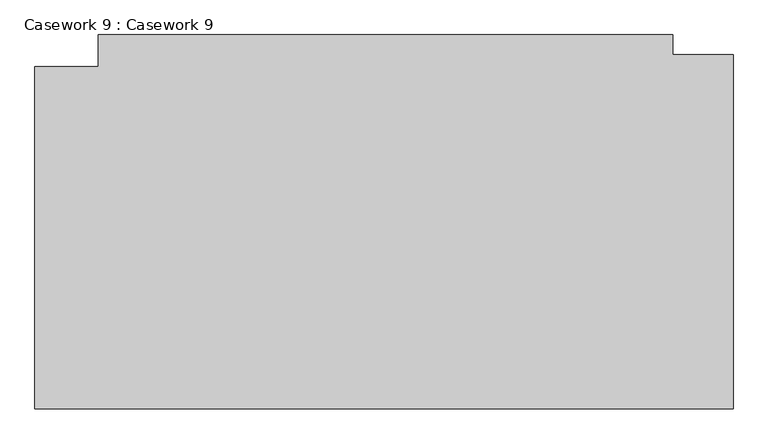
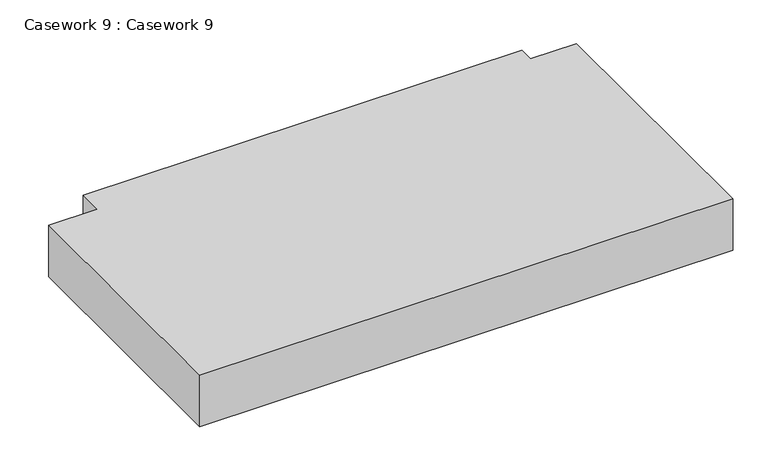
"""IFC4 building model written with IfcOpenShell, lengths in millimetres: furniture geometry, Casework 9 : Casework 9."""

from ifc_helpers import new_model, si_unit, frame, origin, place, context, project, spatial, polyline, outline, extrude, source, transform, mapped, element, save


def casework_9_casework_9_4f7e3acd(model_context):
    return source(origin(), model_context, "Body", "SweptSolid", [
        extrude(outline(polyline([(-7163.5247381, -439.3850684), (-7163.5247381, -339.3850684), (-5353.5247381, -339.3850684), (-5353.5247381, -401.8265396), (-5163.5247381, -401.8265396), (-5163.5247381, -1518.8048922), (-7363.5247381, -1518.8048922), (-7363.5247381, -439.3850684), (-7163.5247381, -439.3850684)])), frame((0.0, 0.0, -225.0091615), z_axis=(0.0, 0.0, 1.0), x_axis=(1.0, 0.0, 0.0)), (0.0, 0.0, 1.0), 225.0091615),
    ])


if __name__ == "__main__":
    model = new_model("IFC4")
    model_context = context("Model", 3, world=origin())
    ifc_project = project(units=[si_unit("LENGTHUNIT", "METRE", prefix="MILLI")], contexts=[model_context])
    site = spatial("IfcSite", under=ifc_project)
    building = spatial("IfcBuilding", under=site)
    placement = place(None, origin())
    casework_9_casework_9_shape = casework_9_casework_9_4f7e3acd(model_context)
    element("IfcFurniture", 1, ObjectType="Casework 9 : Casework 9", at=placement, inside=building, context=model_context, shape_type="MappedRepresentation", body=[
        mapped(casework_9_casework_9_shape, transform((0.0, 0.0, 0.0), x_axis=(1.0, 0.0, 0.0), y_axis=(0.0, 1.0, 0.0), z_axis=(0.0, 0.0, 1.0))),
    ])
    save(model, "model.ifc")

# Revit data of these elements
# Element 1 (IfcFurniture, "Casework 9 : Casework 9")
#   Materials on its faces: "Brick, Common, Brown"
# Materials
#   "Brick, Common, Brown": class "Masonry", colour RGB 153 77 0, transparency 0, Description = "Common brick, brown", Cost = 0
